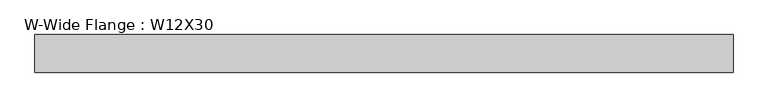
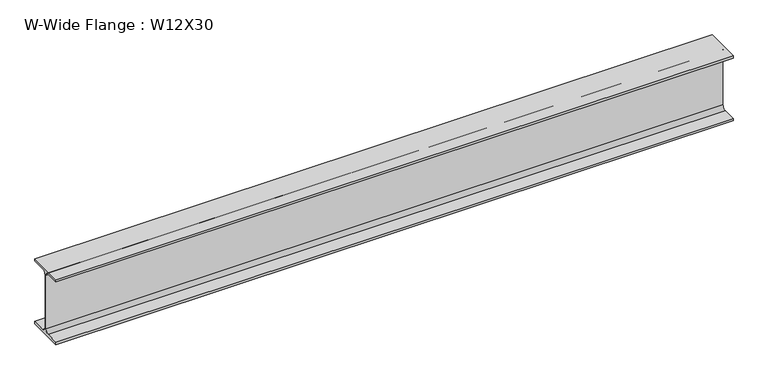
"""IFC4 building model written with IfcOpenShell, lengths in millimetres: beam geometry, W-Wide Flange : W12X30."""

from ifc_helpers import new_model, si_unit, point, frame, frame_2d, origin, place, context, project, spatial, polyline, circle_curve, trimmed, segment, composite_curve, outline, extrude, source, transform, mapped, element, save


def w_wide_flange_w12x30_b48d1e93(model_context):
    return source(origin(), model_context, "Body", "SweptSolid", [
        extrude(outline(composite_curve([segment(polyline([(82.804, -145.034), (82.804, -156.21), (-82.804, -156.21), (-82.804, -145.034), (-20.701, -145.034)]), True, "CONTINUOUS"), segment(trimmed(circle_curve(frame_2d((-20.701, -127.635)), 17.399), [point((-20.701, -145.034))], [point((-3.302, -127.635))], True, "CARTESIAN"), True, "CONTINUOUS"), segment(polyline([(-3.302, -127.635), (-3.302, 127.635)]), True, "CONTINUOUS"), segment(trimmed(circle_curve(frame_2d((-20.701, 127.635)), 17.399), [point((-3.302, 127.635))], [point((-20.701, 145.034))], True, "CARTESIAN"), True, "CONTINUOUS"), segment(polyline([(-20.701, 145.034), (-82.804, 145.034), (-82.804, 156.21), (82.804, 156.21), (82.804, 145.034), (20.701, 145.034)]), True, "CONTINUOUS"), segment(trimmed(circle_curve(frame_2d((20.701, 127.635)), 17.399), [point((20.701, 145.034))], [point((3.302, 127.635))], True, "CARTESIAN"), True, "CONTINUOUS"), segment(polyline([(3.302, 127.635), (3.302, -127.635)]), True, "CONTINUOUS"), segment(trimmed(circle_curve(frame_2d((20.701, -127.635)), 17.399), [point((3.302, -127.635))], [point((20.701, -145.034))], True, "CARTESIAN"), True, "CONTINUOUS"), segment(polyline([(20.701, -145.034), (82.804, -145.034)]), True, "CONTINUOUS")], self_intersect=False)), frame((-1537.4441406, 0.0, 0.0), z_axis=(1.0, 0.0, 0.0), x_axis=(0.0, 1.0, 0.0)), (0.0, 0.0, 1.0), 3074.8882813),
    ])


if __name__ == "__main__":
    model = new_model("IFC4")
    model_context = context("Model", 3, world=origin())
    ifc_project = project(units=[si_unit("LENGTHUNIT", "METRE", prefix="MILLI")], contexts=[model_context])
    site = spatial("IfcSite", under=ifc_project)
    building = spatial("IfcBuilding", under=site)
    placement = place(None, origin())
    w_wide_flange_w12x30_shape = w_wide_flange_w12x30_b48d1e93(model_context)
    element("IfcBeam", 1, ObjectType="W-Wide Flange : W12X30", at=placement, inside=building, context=model_context, shape_type="MappedRepresentation", body=[
        mapped(w_wide_flange_w12x30_shape, transform((0.0, 0.0, 0.0), x_axis=(1.0, 0.0, 0.0), y_axis=(0.0, 1.0, 0.0), z_axis=(0.0, 0.0, 1.0))),
    ])
    save(model, "model.ifc")

# Revit data of these elements
# Type "W-Wide Flange : W12X30"
#   Assembly Code = "B10"
#   W = 30
#   Length [instance default] = 1524 mm
#   bf = 165.608 mm
#   d = 312.42 mm
#   k = 28.575 mm
#   k2 = 17.399 mm
#   tf = 11.176 mm
#   tw = 6.604 mm
#   A = 0.00567096 m²
#   Structural Material [instance default] = Steel ASTM A992
# Element 1 (IfcBeam, "W-Wide Flange : W12X30")
#   Structural Material = Aluminum, Anodized Red
#   Materials on its faces: "Aluminum, Anodized Red"
# Materials
#   "Steel ASTM A992": class "Metal", colour RGB 128 0 0, transparency 0, Description = "Structural steel 50ksi", Cost = 0
#   "Aluminum, Anodized Red": class "Metal", colour RGB 120 120 120, transparency 0, Description = "Anodized aluminum, red", Cost = 0
